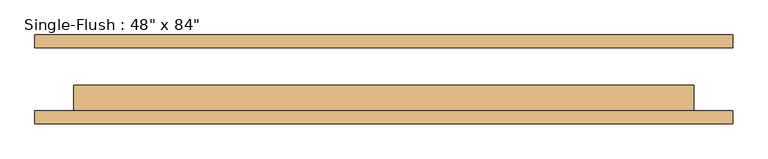
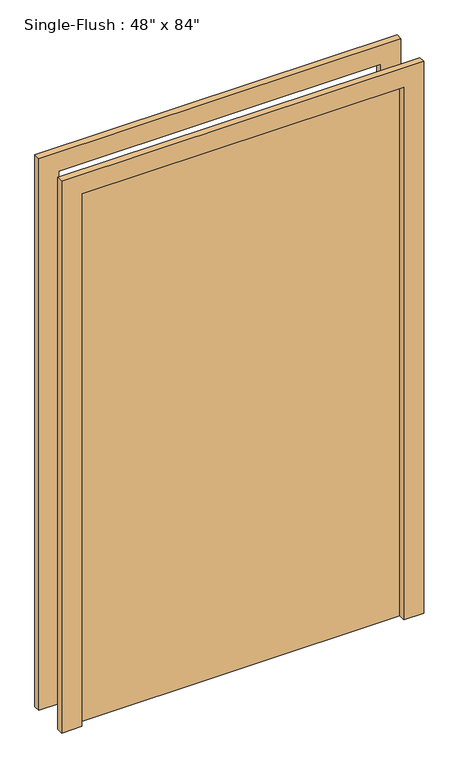
"""IFC4 building model written with IfcOpenShell, lengths in millimetres: door geometry."""

import ifcopenshell
import ifcopenshell.guid

model = None  # the IFC model being written
_history = None  # IfcOwnerHistory: only IFC2X3 demands one
_inside = {}  # id of a spatial element -> (the spatial element, [elements in it])
_under = {}  # id of a project, library or spatial element -> (it, [spatial elements below it])
_declared = {}  # id of a project -> (the project, [libraries it declares])
_typed = {}  # id of a type object -> (the type object, [elements of that type])
_made_of = {}  # id of a material, layer set ... -> (it, [elements and type objects made of it])


def new_model(schema):
    """Start an empty IFC model of exactly this schema.

    Asked for "IFC4X3", IfcOpenShell would pick the latest addendum, in which some entities
    have other attributes; the version numbers below select the first issue.
    IFC2X3 requires an IfcOwnerHistory on every rooted entity: one is made here for all.
    """
    global model, _history
    if schema == "IFC4X3":
        model = ifcopenshell.file(schema_version=(4, 3, 0, 0))
    else:
        model = ifcopenshell.file(schema=schema)
    _inside.clear()
    _under.clear()
    _declared.clear()
    _typed.clear()
    _made_of.clear()
    _history = None
    if model.schema == "IFC2X3":
        org = make("IfcOrganization", Name="unknown")
        user = make(
            "IfcPersonAndOrganization",
            ThePerson=make("IfcPerson", FamilyName="unknown"),
            TheOrganization=org,
        )
        app = make(
            "IfcApplication",
            ApplicationDeveloper=org,
            Version="unknown",
            ApplicationFullName="unknown",
            ApplicationIdentifier="unknown",
        )
        _history = make(
            "IfcOwnerHistory",
            OwningUser=user,
            OwningApplication=app,
            ChangeAction="ADDED",
            CreationDate=0,
        )
    return model


def make(cls, **values):
    """One entity of the class cls with the attributes given. An attribute that is None is left unset."""
    return model.create_entity(
        cls, **{name: value for name, value in values.items() if value is not None}
    )


def rooted(cls, **values):
    """An entity with a GlobalId (a new one), such as an element, a storey or a relation."""
    return make(cls, GlobalId=ifcopenshell.guid.new(), OwnerHistory=_history, **values)


def si_unit(unit_type, name, prefix=None):
    """IfcSIUnit, for example si_unit("LENGTHUNIT", "METRE", prefix="MILLI")."""
    return make("IfcSIUnit", UnitType=unit_type, Prefix=prefix, Name=name)


def assignment(units):
    """IfcUnitAssignment: the units of a project."""
    return None if units is None else make("IfcUnitAssignment", Units=units)


def point(xyz):
    """IfcCartesianPoint."""
    return None if xyz is None else make("IfcCartesianPoint", Coordinates=xyz)


def direction(xyz):
    """IfcDirection."""
    return None if xyz is None else make("IfcDirection", DirectionRatios=xyz)


def frame(location, z_axis=None, x_axis=None):
    """IfcAxis2Placement3D, a coordinate frame: its origin and axes. An axis left out is left unset."""
    return make(
        "IfcAxis2Placement3D",
        Location=point(location),
        Axis=direction(z_axis),
        RefDirection=direction(x_axis),
    )


def origin():
    """The frame at (0, 0, 0) with its axes left unset."""
    return frame((0.0, 0.0, 0.0))


def origin_with_axes():
    """The frame at (0, 0, 0) with the z axis (0, 0, 1) and the x axis (1, 0, 0) written out."""
    return frame((0.0, 0.0, 0.0), z_axis=(0.0, 0.0, 1.0), x_axis=(1.0, 0.0, 0.0))


def place(relative_to, where):
    """IfcLocalPlacement: puts the frame where relative to a parent placement (None: the world)."""
    return make(
        "IfcLocalPlacement", PlacementRelTo=relative_to, RelativePlacement=where
    )


def context(
    kind, dimensions, precision=None, world=None, true_north=None, identifier=None
):
    """IfcGeometricRepresentationContext, for example the 3D "Model" context."""
    return make(
        "IfcGeometricRepresentationContext",
        ContextIdentifier=identifier,
        ContextType=kind,
        CoordinateSpaceDimension=dimensions,
        Precision=precision,
        WorldCoordinateSystem=world,
        TrueNorth=true_north,
    )


def project(units=None, contexts=None):
    """IfcProject with its units and contexts."""
    return rooted(
        "IfcProject",
        Name="project",
        RepresentationContexts=contexts,
        UnitsInContext=assignment(units),
    )


def spatial(cls, under=None, at=None, **own):
    """A site, building, storey or space (cls), placed at a placement, below another one or the project."""
    s = rooted(cls, ObjectPlacement=at, **own)
    if under is not None:
        _under.setdefault(under.id(), (under, []))[1].append(s)
    return s


def polyline(points):
    """IfcPolyline through the points."""
    return make("IfcPolyline", Points=[point(p) for p in points])


def outline(outer, holes=None, kind="AREA"):
    """IfcArbitraryClosedProfileDef: a profile drawn as a closed curve; with holes, ...WithVoids."""
    if holes is None:
        return make("IfcArbitraryClosedProfileDef", ProfileType=kind, OuterCurve=outer)
    return make(
        "IfcArbitraryProfileDefWithVoids",
        ProfileType=kind,
        OuterCurve=outer,
        InnerCurves=holes,
    )


def extrude(swept, where, along, depth):
    """IfcExtrudedAreaSolid: the profile swept, set in the frame where, extruded along a direction by depth."""
    return make(
        "IfcExtrudedAreaSolid",
        SweptArea=swept,
        Position=where,
        ExtrudedDirection=direction(along),
        Depth=depth,
    )


def shape(context_of_items, identifier, shape_type, items):
    """IfcShapeRepresentation: the items that make up one representation, for example the "Body"."""
    return make(
        "IfcShapeRepresentation",
        ContextOfItems=context_of_items,
        RepresentationIdentifier=identifier,
        RepresentationType=shape_type,
        Items=items,
    )


def source(mapping_origin, context_of_items, identifier, shape_type, items):
    """IfcRepresentationMap: a shape defined once, which mapped items show again and again."""
    return make(
        "IfcRepresentationMap",
        MappingOrigin=mapping_origin,
        MappedRepresentation=shape(context_of_items, identifier, shape_type, items),
    )


def transform(
    local_origin,
    x_axis=None,
    y_axis=None,
    z_axis=None,
    scale=None,
    scale2=None,
    scale3=None,
    uniform=True,
):
    """IfcCartesianTransformationOperator3D, or its non-uniform kind. x_axis, y_axis, z_axis: its Axis1, 2, 3."""
    if uniform:
        return make(
            "IfcCartesianTransformationOperator3D",
            Axis1=direction(x_axis),
            Axis2=direction(y_axis),
            LocalOrigin=point(local_origin),
            Scale=scale,
            Axis3=direction(z_axis),
        )
    return make(
        "IfcCartesianTransformationOperator3DnonUniform",
        Axis1=direction(x_axis),
        Axis2=direction(y_axis),
        LocalOrigin=point(local_origin),
        Scale=scale,
        Axis3=direction(z_axis),
        Scale2=scale2,
        Scale3=scale3,
    )


def mapped(mapping_source, mapping_target):
    """IfcMappedItem: shows the shape of a source again, moved by a transform."""
    return make(
        "IfcMappedItem", MappingSource=mapping_source, MappingTarget=mapping_target
    )


def made_of(thing, what):
    """Note that an element or type object is made of a material, layer set ...; save() writes the relation."""
    if what is not None:
        _made_of.setdefault(what.id(), (what, []))[1].append(thing)
    return thing


def element(
    cls,
    number,
    at=None,
    inside=None,
    cuts=None,
    type_object=None,
    material=None,
    context=None,
    identifier="Body",
    shape_type=None,
    held_by="IfcProductDefinitionShape",
    body=None,
    shapes=None,
    **own,
):
    """One element of the class cls, such as IfcWall. Its Tag is "e" and its number.

    at: its placement. inside: the storey or other place that contains it. cuts: it is an
    opening in that element (IfcRelVoidsElement). A single representation is given by context,
    identifier, shape_type and body (its items); several are given by shapes. held_by: the class
    of the entity that holds the representations. save() writes the other relations.
    """
    e = rooted(cls, Tag="e%d" % number, ObjectPlacement=at, **own)
    if body is not None:
        shapes = [shape(context, identifier, shape_type, body)]
    if shapes is not None:
        e.Representation = make(held_by, Representations=shapes)
    if inside is not None:
        _inside.setdefault(inside.id(), (inside, []))[1].append(e)
    if cuts is not None:
        rooted(
            "IfcRelVoidsElement", RelatingBuildingElement=cuts, RelatedOpeningElement=e
        )
    if type_object is not None:
        _typed.setdefault(type_object.id(), (type_object, []))[1].append(e)
    return made_of(e, material)


def aggregate(whole, parts):
    """IfcRelAggregates: a whole, such as a stair, and the parts it consists of."""
    return rooted("IfcRelAggregates", RelatingObject=whole, RelatedObjects=parts)


def save(model, path):
    """Write the relations noted so far, then the file.

    IfcRelAggregates (storeys below a building ...), IfcRelContainedInSpatialStructure (elements
    in a storey), IfcRelDefinesByType, IfcRelAssociatesMaterial and IfcRelDeclares: one each for
    every whole, place, type object, material and project.
    """
    for whole, parts in _under.values():
        aggregate(whole, parts)
    for where, things in _inside.values():
        rooted(
            "IfcRelContainedInSpatialStructure",
            RelatedElements=things,
            RelatingStructure=where,
        )
    for kind, things in _typed.values():
        rooted("IfcRelDefinesByType", RelatedObjects=things, RelatingType=kind)
    for what, things in _made_of.values():
        rooted("IfcRelAssociatesMaterial", RelatedObjects=things, RelatingMaterial=what)
    for by, libraries in _declared.values():
        rooted("IfcRelDeclares", RelatingContext=by, RelatedDefinitions=libraries)
    model.write(path)


def door_1f4748c7(model_context):
    return source(origin(), model_context, "Body", "SweptSolid", [
        extrude(outline(polyline([(2209.8, -685.8), (0.0, -685.8), (0.0, -609.6), (2133.6, -609.6), (2133.6, 609.6), (0.0, 609.6), (0.0, 685.8), (2209.8, 685.8), (2209.8, -685.8)])), frame((0.0, -87.3125, 0.0), z_axis=(0.0, 1.0, 0.0), x_axis=(0.0, 0.0, 1.0)), (0.0, 0.0, 1.0), 25.4),
        extrude(outline(polyline([(2209.8, 685.8), (2209.8, -685.8), (0.0, -685.8), (0.0, -609.6), (2133.6, -609.6), (2133.6, 609.6), (0.0, 609.6), (0.0, 685.8), (2209.8, 685.8)])), frame((0.0, 61.9125, 0.0), z_axis=(0.0, 1.0, 0.0), x_axis=(0.0, 0.0, 1.0)), (0.0, 0.0, 1.0), 25.4),
        extrude(outline(polyline([(609.6, -11.1125), (609.6, -61.9125), (-609.6, -61.9125), (-609.6, -11.1125), (609.6, -11.1125)])), origin_with_axes(), (0.0, 0.0, 1.0), 2133.6),
    ])


if __name__ == "__main__":
    model = new_model("IFC4")
    model_context = context("Model", 3, world=origin())
    ifc_project = project(units=[si_unit("LENGTHUNIT", "METRE", prefix="MILLI")], contexts=[model_context])
    site = spatial("IfcSite", under=ifc_project)
    building = spatial("IfcBuilding", under=site)
    placement = place(None, origin())
    door_shape = door_1f4748c7(model_context)
    element("IfcDoor", 1, ObjectType="Single-Flush : 48\" x 84\"", at=placement, inside=building, context=model_context, shape_type="MappedRepresentation", body=[
        mapped(door_shape, transform((0.0, 0.0, 0.0), x_axis=(1.0, 0.0, 0.0), y_axis=(0.0, 1.0, 0.0), z_axis=(0.0, 0.0, 1.0))),
    ])
    save(model, "model.ifc")

# Revit data of these elements
# Type "Single-Flush : 48\" x 84\""
#   Type Mark = "8"
#   Construction Type = "C"
#   Assembly Code = "C1020"
#   Thickness = 0' - 2"
#   Height = 7' - 0"
#   Trim Projection Ext = 0' - 1"
#   Trim Projection Int = 0' - 1"
#   Trim Width = 0' - 3"
#   Width = 4' - 0"
#   Door Material = Door - Panel
#   Frame Material = Door - Frame
#   Function = (empty or 0)
#   Wall Closure = (empty or 0)
# Element 1 (IfcDoor, "Single-Flush : 48\" x 84\"")
#   Materials on its faces: "Door - Frame", "Door - Panel"
# Materials
#   "Door - Panel": class "Wood", colour RGB 210 159 95, transparency 0
#   "Door - Frame": class "Miscellaneous", colour RGB 118 70 51, transparency 0
